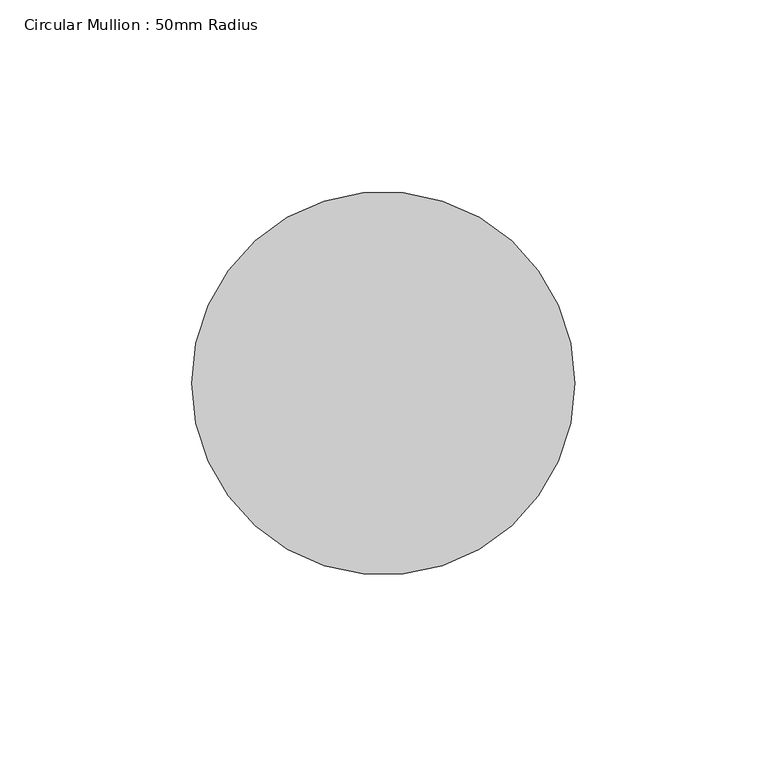
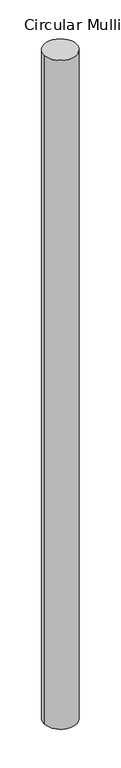
"""IFC4 building model written with IfcOpenShell, lengths in millimetres: member geometry, Circular Mullion : 50mm Radius."""

from ifc_helpers import new_model, si_unit, point, frame, origin, origin_2d, place, context, project, spatial, circle_curve, trimmed, segment, composite_curve, outline, extrude, source, transform, mapped, element, save


def circular_mullion_50mm_radius_702b3722(model_context):
    return source(origin(), model_context, "Body", "SweptSolid", [
        extrude(outline(composite_curve([segment(trimmed(circle_curve(origin_2d(), 50.0), [point((50.0, 0.0))], [point((-50.0, 0.0))], False, "CARTESIAN"), True, "CONTINUOUS"), segment(trimmed(circle_curve(origin_2d(), 50.0), [point((-50.0, 0.0))], [point((50.0, 0.0))], False, "CARTESIAN"), True, "CONTINUOUS")], self_intersect=False)), frame((0.0, 0.0, -2164.8381989), z_axis=(0.0, 0.0, 1.0), x_axis=(1.0, 0.0, 0.0)), (0.0, 0.0, 1.0), 2164.8381989),
    ])


if __name__ == "__main__":
    model = new_model("IFC4")
    model_context = context("Model", 3, world=origin())
    ifc_project = project(units=[si_unit("LENGTHUNIT", "METRE", prefix="MILLI")], contexts=[model_context])
    site = spatial("IfcSite", under=ifc_project)
    building = spatial("IfcBuilding", under=site)
    placement = place(None, origin())
    circular_mullion_50mm_radius_shape = circular_mullion_50mm_radius_702b3722(model_context)
    element("IfcMember", 1, ObjectType="Circular Mullion : 50mm Radius", at=placement, inside=building, context=model_context, shape_type="MappedRepresentation", body=[
        mapped(circular_mullion_50mm_radius_shape, transform((0.0, 0.0, 0.0), x_axis=(1.0, 0.0, 0.0), y_axis=(0.0, 1.0, 0.0), z_axis=(0.0, 0.0, 1.0))),
    ])
    save(model, "model.ifc")

# Revit data of these elements
# Type "Circular Mullion : 50mm Radius"
#   built-in parameter 1007350 = 0.164042 (stored number, unit not read)
# Element 1 (IfcMember, "Circular Mullion : 50mm Radius")
#   Materials on its faces: "Aluminium"
# Materials
#   "Aluminium": class "Metal", colour RGB 247 247 247, transparency 0, Description = "Aluminium 6061", Cost = 0
